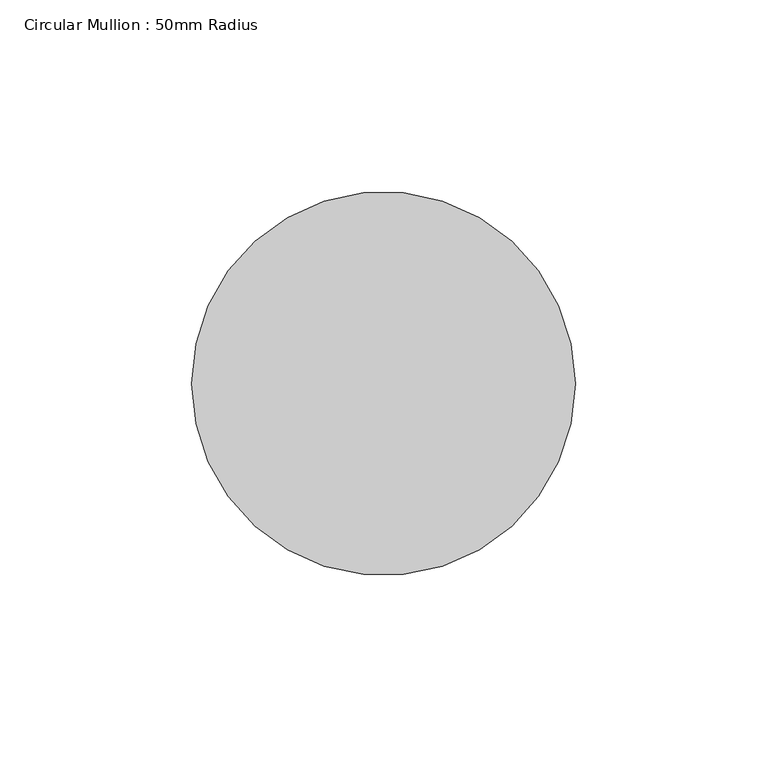
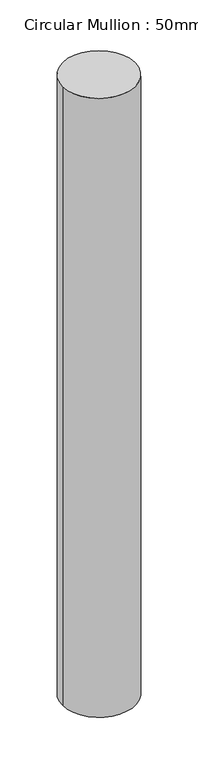
"""IFC4 building model written with IfcOpenShell, lengths in millimetres: member geometry, Circular Mullion : 50mm Radius."""

import ifcopenshell
import ifcopenshell.guid

model = None  # the IFC model being written
_history = None  # IfcOwnerHistory: only IFC2X3 demands one
_inside = {}  # id of a spatial element -> (the spatial element, [elements in it])
_under = {}  # id of a project, library or spatial element -> (it, [spatial elements below it])
_declared = {}  # id of a project -> (the project, [libraries it declares])
_typed = {}  # id of a type object -> (the type object, [elements of that type])
_made_of = {}  # id of a material, layer set ... -> (it, [elements and type objects made of it])


def new_model(schema):
    """Start an empty IFC model of exactly this schema.

    Asked for "IFC4X3", IfcOpenShell would pick the latest addendum, in which some entities
    have other attributes; the version numbers below select the first issue.
    IFC2X3 requires an IfcOwnerHistory on every rooted entity: one is made here for all.
    """
    global model, _history
    if schema == "IFC4X3":
        model = ifcopenshell.file(schema_version=(4, 3, 0, 0))
    else:
        model = ifcopenshell.file(schema=schema)
    _inside.clear()
    _under.clear()
    _declared.clear()
    _typed.clear()
    _made_of.clear()
    _history = None
    if model.schema == "IFC2X3":
        org = make("IfcOrganization", Name="unknown")
        user = make(
            "IfcPersonAndOrganization",
            ThePerson=make("IfcPerson", FamilyName="unknown"),
            TheOrganization=org,
        )
        app = make(
            "IfcApplication",
            ApplicationDeveloper=org,
            Version="unknown",
            ApplicationFullName="unknown",
            ApplicationIdentifier="unknown",
        )
        _history = make(
            "IfcOwnerHistory",
            OwningUser=user,
            OwningApplication=app,
            ChangeAction="ADDED",
            CreationDate=0,
        )
    return model


def make(cls, **values):
    """One entity of the class cls with the attributes given. An attribute that is None is left unset."""
    return model.create_entity(
        cls, **{name: value for name, value in values.items() if value is not None}
    )


def rooted(cls, **values):
    """An entity with a GlobalId (a new one), such as an element, a storey or a relation."""
    return make(cls, GlobalId=ifcopenshell.guid.new(), OwnerHistory=_history, **values)


def si_unit(unit_type, name, prefix=None):
    """IfcSIUnit, for example si_unit("LENGTHUNIT", "METRE", prefix="MILLI")."""
    return make("IfcSIUnit", UnitType=unit_type, Prefix=prefix, Name=name)


def assignment(units):
    """IfcUnitAssignment: the units of a project."""
    return None if units is None else make("IfcUnitAssignment", Units=units)


def point(xyz):
    """IfcCartesianPoint."""
    return None if xyz is None else make("IfcCartesianPoint", Coordinates=xyz)


def direction(xyz):
    """IfcDirection."""
    return None if xyz is None else make("IfcDirection", DirectionRatios=xyz)


def frame(location, z_axis=None, x_axis=None):
    """IfcAxis2Placement3D, a coordinate frame: its origin and axes. An axis left out is left unset."""
    return make(
        "IfcAxis2Placement3D",
        Location=point(location),
        Axis=direction(z_axis),
        RefDirection=direction(x_axis),
    )


def frame_2d(location, x_axis=None):
    """IfcAxis2Placement2D, a coordinate frame in the plane: its origin and x axis."""
    return make(
        "IfcAxis2Placement2D", Location=point(location), RefDirection=direction(x_axis)
    )


def origin():
    """The frame at (0, 0, 0) with its axes left unset."""
    return frame((0.0, 0.0, 0.0))


def origin_2d():
    """The frame at (0, 0) in the plane with its x axis left unset."""
    return frame_2d((0.0, 0.0))


def place(relative_to, where):
    """IfcLocalPlacement: puts the frame where relative to a parent placement (None: the world)."""
    return make(
        "IfcLocalPlacement", PlacementRelTo=relative_to, RelativePlacement=where
    )


def context(
    kind, dimensions, precision=None, world=None, true_north=None, identifier=None
):
    """IfcGeometricRepresentationContext, for example the 3D "Model" context."""
    return make(
        "IfcGeometricRepresentationContext",
        ContextIdentifier=identifier,
        ContextType=kind,
        CoordinateSpaceDimension=dimensions,
        Precision=precision,
        WorldCoordinateSystem=world,
        TrueNorth=true_north,
    )


def project(units=None, contexts=None):
    """IfcProject with its units and contexts."""
    return rooted(
        "IfcProject",
        Name="project",
        RepresentationContexts=contexts,
        UnitsInContext=assignment(units),
    )


def spatial(cls, under=None, at=None, **own):
    """A site, building, storey or space (cls), placed at a placement, below another one or the project."""
    s = rooted(cls, ObjectPlacement=at, **own)
    if under is not None:
        _under.setdefault(under.id(), (under, []))[1].append(s)
    return s


def circle_curve(where, radius):
    """IfcCircle in the frame where."""
    return make("IfcCircle", Position=where, Radius=radius)


def trimmed(basis, trim1, trim2, sense, master):
    """IfcTrimmedCurve: the piece of a basis curve between two trims."""
    return make(
        "IfcTrimmedCurve",
        BasisCurve=basis,
        Trim1=trim1,
        Trim2=trim2,
        SenseAgreement=sense,
        MasterRepresentation=master,
    )


def segment(curve, same_sense, transition):
    """IfcCompositeCurveSegment."""
    return make(
        "IfcCompositeCurveSegment",
        Transition=transition,
        SameSense=same_sense,
        ParentCurve=curve,
    )


def composite_curve(segments, self_intersect=None):
    """IfcCompositeCurve: segments joined end to end."""
    return make("IfcCompositeCurve", Segments=segments, SelfIntersect=self_intersect)


def outline(outer, holes=None, kind="AREA"):
    """IfcArbitraryClosedProfileDef: a profile drawn as a closed curve; with holes, ...WithVoids."""
    if holes is None:
        return make("IfcArbitraryClosedProfileDef", ProfileType=kind, OuterCurve=outer)
    return make(
        "IfcArbitraryProfileDefWithVoids",
        ProfileType=kind,
        OuterCurve=outer,
        InnerCurves=holes,
    )


def extrude(swept, where, along, depth):
    """IfcExtrudedAreaSolid: the profile swept, set in the frame where, extruded along a direction by depth."""
    return make(
        "IfcExtrudedAreaSolid",
        SweptArea=swept,
        Position=where,
        ExtrudedDirection=direction(along),
        Depth=depth,
    )


def shape(context_of_items, identifier, shape_type, items):
    """IfcShapeRepresentation: the items that make up one representation, for example the "Body"."""
    return make(
        "IfcShapeRepresentation",
        ContextOfItems=context_of_items,
        RepresentationIdentifier=identifier,
        RepresentationType=shape_type,
        Items=items,
    )


def source(mapping_origin, context_of_items, identifier, shape_type, items):
    """IfcRepresentationMap: a shape defined once, which mapped items show again and again."""
    return make(
        "IfcRepresentationMap",
        MappingOrigin=mapping_origin,
        MappedRepresentation=shape(context_of_items, identifier, shape_type, items),
    )


def transform(
    local_origin,
    x_axis=None,
    y_axis=None,
    z_axis=None,
    scale=None,
    scale2=None,
    scale3=None,
    uniform=True,
):
    """IfcCartesianTransformationOperator3D, or its non-uniform kind. x_axis, y_axis, z_axis: its Axis1, 2, 3."""
    if uniform:
        return make(
            "IfcCartesianTransformationOperator3D",
            Axis1=direction(x_axis),
            Axis2=direction(y_axis),
            LocalOrigin=point(local_origin),
            Scale=scale,
            Axis3=direction(z_axis),
        )
    return make(
        "IfcCartesianTransformationOperator3DnonUniform",
        Axis1=direction(x_axis),
        Axis2=direction(y_axis),
        LocalOrigin=point(local_origin),
        Scale=scale,
        Axis3=direction(z_axis),
        Scale2=scale2,
        Scale3=scale3,
    )


def mapped(mapping_source, mapping_target):
    """IfcMappedItem: shows the shape of a source again, moved by a transform."""
    return make(
        "IfcMappedItem", MappingSource=mapping_source, MappingTarget=mapping_target
    )


def made_of(thing, what):
    """Note that an element or type object is made of a material, layer set ...; save() writes the relation."""
    if what is not None:
        _made_of.setdefault(what.id(), (what, []))[1].append(thing)
    return thing


def element(
    cls,
    number,
    at=None,
    inside=None,
    cuts=None,
    type_object=None,
    material=None,
    context=None,
    identifier="Body",
    shape_type=None,
    held_by="IfcProductDefinitionShape",
    body=None,
    shapes=None,
    **own,
):
    """One element of the class cls, such as IfcWall. Its Tag is "e" and its number.

    at: its placement. inside: the storey or other place that contains it. cuts: it is an
    opening in that element (IfcRelVoidsElement). A single representation is given by context,
    identifier, shape_type and body (its items); several are given by shapes. held_by: the class
    of the entity that holds the representations. save() writes the other relations.
    """
    e = rooted(cls, Tag="e%d" % number, ObjectPlacement=at, **own)
    if body is not None:
        shapes = [shape(context, identifier, shape_type, body)]
    if shapes is not None:
        e.Representation = make(held_by, Representations=shapes)
    if inside is not None:
        _inside.setdefault(inside.id(), (inside, []))[1].append(e)
    if cuts is not None:
        rooted(
            "IfcRelVoidsElement", RelatingBuildingElement=cuts, RelatedOpeningElement=e
        )
    if type_object is not None:
        _typed.setdefault(type_object.id(), (type_object, []))[1].append(e)
    return made_of(e, material)


def aggregate(whole, parts):
    """IfcRelAggregates: a whole, such as a stair, and the parts it consists of."""
    return rooted("IfcRelAggregates", RelatingObject=whole, RelatedObjects=parts)


def save(model, path):
    """Write the relations noted so far, then the file.

    IfcRelAggregates (storeys below a building ...), IfcRelContainedInSpatialStructure (elements
    in a storey), IfcRelDefinesByType, IfcRelAssociatesMaterial and IfcRelDeclares: one each for
    every whole, place, type object, material and project.
    """
    for whole, parts in _under.values():
        aggregate(whole, parts)
    for where, things in _inside.values():
        rooted(
            "IfcRelContainedInSpatialStructure",
            RelatedElements=things,
            RelatingStructure=where,
        )
    for kind, things in _typed.values():
        rooted("IfcRelDefinesByType", RelatedObjects=things, RelatingType=kind)
    for what, things in _made_of.values():
        rooted("IfcRelAssociatesMaterial", RelatedObjects=things, RelatingMaterial=what)
    for by, libraries in _declared.values():
        rooted("IfcRelDeclares", RelatingContext=by, RelatedDefinitions=libraries)
    model.write(path)


def circular_mullion_50mm_radius_6f785a31(model_context):
    return source(origin(), model_context, "Body", "SweptSolid", [
        extrude(outline(composite_curve([segment(trimmed(circle_curve(origin_2d(), 50.0), [point((50.0, 0.0))], [point((-50.0, 0.0))], False, "CARTESIAN"), True, "CONTINUOUS"), segment(trimmed(circle_curve(origin_2d(), 50.0), [point((-50.0, 0.0))], [point((50.0, 0.0))], False, "CARTESIAN"), True, "CONTINUOUS")], self_intersect=False)), frame((0.0, 0.0, -904.0507455), z_axis=(0.0, 0.0, 1.0), x_axis=(1.0, 0.0, 0.0)), (0.0, 0.0, 1.0), 904.0507455),
    ])


if __name__ == "__main__":
    model = new_model("IFC4")
    model_context = context("Model", 3, world=origin())
    ifc_project = project(units=[si_unit("LENGTHUNIT", "METRE", prefix="MILLI")], contexts=[model_context])
    site = spatial("IfcSite", under=ifc_project)
    building = spatial("IfcBuilding", under=site)
    placement = place(None, origin())
    circular_mullion_50mm_radius_shape = circular_mullion_50mm_radius_6f785a31(model_context)
    element("IfcMember", 1, ObjectType="Circular Mullion : 50mm Radius", at=placement, inside=building, context=model_context, shape_type="MappedRepresentation", body=[
        mapped(circular_mullion_50mm_radius_shape, transform((0.0, 0.0, 0.0), x_axis=(1.0, 0.0, 0.0), y_axis=(0.0, 1.0, 0.0), z_axis=(0.0, 0.0, 1.0))),
    ])
    save(model, "model.ifc")

# Revit data of these elements
# Type "Circular Mullion : 50mm Radius"
#   built-in parameter 1007350 = 0.164042 (stored number, unit not read)
# Element 1 (IfcMember, "Circular Mullion : 50mm Radius")
#   Materials on its faces: "Aluminium"
# Materials
#   "Aluminium": class "Metal", colour RGB 247 247 247, transparency 0, Description = "Aluminium 6061", Cost = 0
